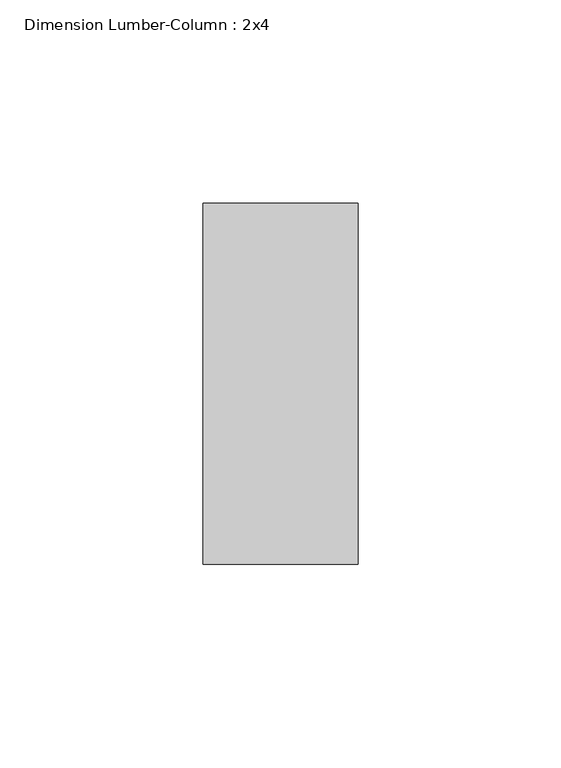
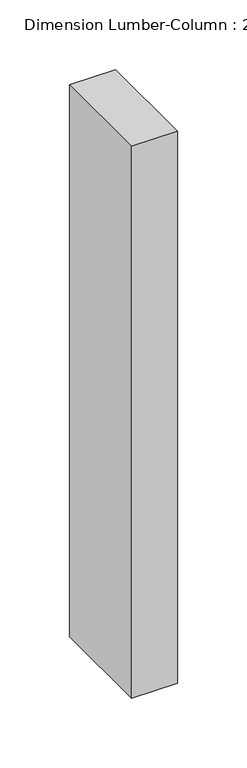
"""IFC4 building model written with IfcOpenShell, lengths in millimetres: column geometry, Dimension Lumber-Column : 2x4."""

from ifc_helpers import new_model, si_unit, frame, origin, place, context, project, spatial, polyline, outline, extrude, source, transform, mapped, element, save


def dimension_lumber_column_2x4_c2f848da(model_context):
    return source(origin(), model_context, "Body", "SweptSolid", [
        extrude(outline(polyline([(19.05, 44.45), (19.05, -44.45), (-19.05, -44.45), (-19.05, 44.45), (19.05, 44.45)])), frame((0.0, 0.0, 2208.609375), z_axis=(0.0, 0.0, 1.0), x_axis=(1.0, 0.0, 0.0)), (0.0, 0.0, 1.0), 483.790625),
    ])


if __name__ == "__main__":
    model = new_model("IFC4")
    model_context = context("Model", 3, world=origin())
    ifc_project = project(units=[si_unit("LENGTHUNIT", "METRE", prefix="MILLI")], contexts=[model_context])
    site = spatial("IfcSite", under=ifc_project)
    building = spatial("IfcBuilding", under=site)
    placement = place(None, origin())
    dimension_lumber_column_2x4_shape = dimension_lumber_column_2x4_c2f848da(model_context)
    element("IfcColumn", 1, ObjectType="Dimension Lumber-Column : 2x4", at=placement, inside=building, context=model_context, shape_type="MappedRepresentation", body=[
        mapped(dimension_lumber_column_2x4_shape, transform((0.0, 0.0, 0.0), x_axis=(1.0, 0.0, 0.0), y_axis=(0.0, 1.0, 0.0), z_axis=(0.0, 0.0, 1.0))),
    ])
    save(model, "model.ifc")

# Revit data of these elements
# Type "Dimension Lumber-Column : 2x4"
#   Int Type = "Interior"
#   Assembly Code = "B10"
#   Cost = 8.05
#   A = 0.0364583 SF
#   b = 0' - 1 1/2"
#   d = 0' - 3 1/2"
#   Structural Material [instance default] = Softwood, Lumber
# Element 1 (IfcColumn, "Dimension Lumber-Column : 2x4")
#   Structural Material = Douglas Fir #2
#   Materials on its faces: "Douglas Fir #2"
# Materials
#   "Softwood, Lumber": class "Wood", colour RGB 223 192 134, transparency 0, Description = "Pinus Echinata", Cost = 0
#   "Douglas Fir #2": class "Wood", colour RGB 223 192 134, transparency 0, Description = "Pinus Echinata", Cost = 0
